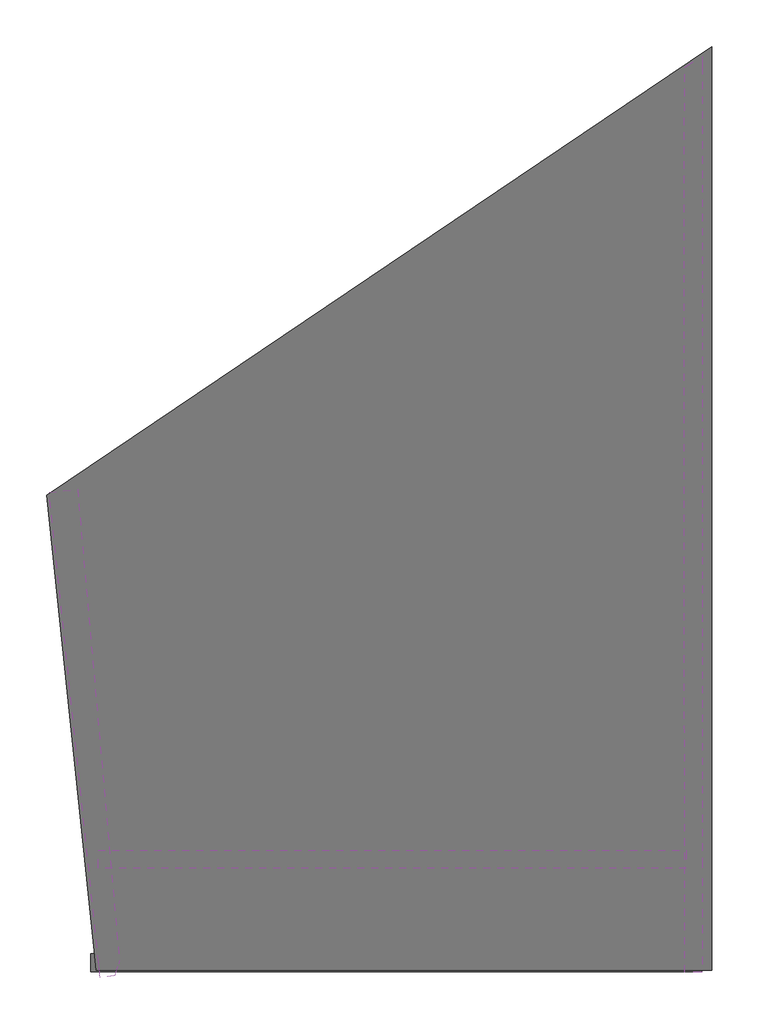
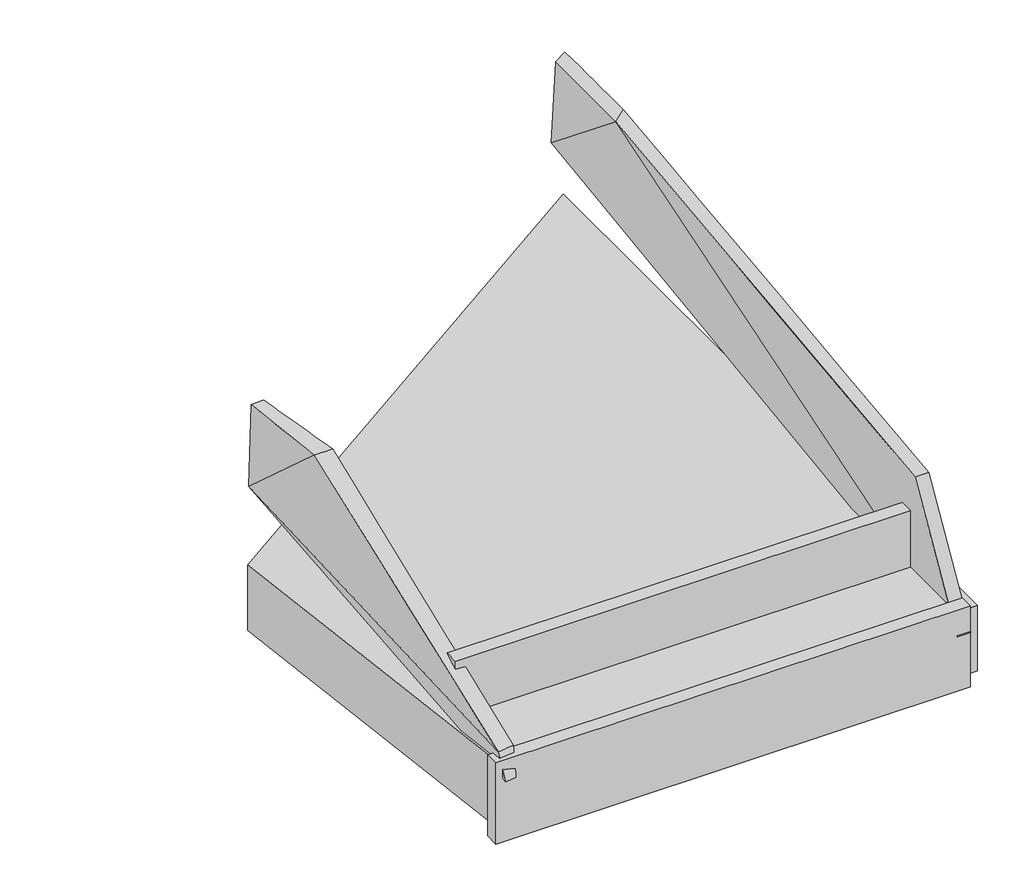
# One storey: 5 proxies.
"""IFC4 building model written with IfcOpenShell, lengths in millimetres."""

import ifcopenshell
import ifcopenshell.guid

model = None  # the IFC model being written
_history = None  # IfcOwnerHistory: only IFC2X3 demands one
_inside = {}  # id of a spatial element -> (the spatial element, [elements in it])
_under = {}  # id of a project, library or spatial element -> (it, [spatial elements below it])
_declared = {}  # id of a project -> (the project, [libraries it declares])
_typed = {}  # id of a type object -> (the type object, [elements of that type])
_made_of = {}  # id of a material, layer set ... -> (it, [elements and type objects made of it])


def new_model(schema):
    """Start an empty IFC model of exactly this schema.

    Asked for "IFC4X3", IfcOpenShell would pick the latest addendum, in which some entities
    have other attributes; the version numbers below select the first issue.
    IFC2X3 requires an IfcOwnerHistory on every rooted entity: one is made here for all.
    """
    global model, _history
    if schema == "IFC4X3":
        model = ifcopenshell.file(schema_version=(4, 3, 0, 0))
    else:
        model = ifcopenshell.file(schema=schema)
    _inside.clear()
    _under.clear()
    _declared.clear()
    _typed.clear()
    _made_of.clear()
    _history = None
    if model.schema == "IFC2X3":
        org = make("IfcOrganization", Name="unknown")
        user = make(
            "IfcPersonAndOrganization",
            ThePerson=make("IfcPerson", FamilyName="unknown"),
            TheOrganization=org,
        )
        app = make(
            "IfcApplication",
            ApplicationDeveloper=org,
            Version="unknown",
            ApplicationFullName="unknown",
            ApplicationIdentifier="unknown",
        )
        _history = make(
            "IfcOwnerHistory",
            OwningUser=user,
            OwningApplication=app,
            ChangeAction="ADDED",
            CreationDate=0,
        )
    return model


def make(cls, **values):
    """One entity of the class cls with the attributes given. An attribute that is None is left unset."""
    return model.create_entity(
        cls, **{name: value for name, value in values.items() if value is not None}
    )


def rooted(cls, **values):
    """An entity with a GlobalId (a new one), such as an element, a storey or a relation."""
    return make(cls, GlobalId=ifcopenshell.guid.new(), OwnerHistory=_history, **values)


def si_unit(unit_type, name, prefix=None):
    """IfcSIUnit, for example si_unit("LENGTHUNIT", "METRE", prefix="MILLI")."""
    return make("IfcSIUnit", UnitType=unit_type, Prefix=prefix, Name=name)


def assignment(units):
    """IfcUnitAssignment: the units of a project."""
    return None if units is None else make("IfcUnitAssignment", Units=units)


def point(xyz):
    """IfcCartesianPoint."""
    return None if xyz is None else make("IfcCartesianPoint", Coordinates=xyz)


def direction(xyz):
    """IfcDirection."""
    return None if xyz is None else make("IfcDirection", DirectionRatios=xyz)


def frame(location, z_axis=None, x_axis=None):
    """IfcAxis2Placement3D, a coordinate frame: its origin and axes. An axis left out is left unset."""
    return make(
        "IfcAxis2Placement3D",
        Location=point(location),
        Axis=direction(z_axis),
        RefDirection=direction(x_axis),
    )


def origin():
    """The frame at (0, 0, 0) with its axes left unset."""
    return frame((0.0, 0.0, 0.0))


def place(relative_to, where):
    """IfcLocalPlacement: puts the frame where relative to a parent placement (None: the world)."""
    return make(
        "IfcLocalPlacement", PlacementRelTo=relative_to, RelativePlacement=where
    )


def context(
    kind, dimensions, precision=None, world=None, true_north=None, identifier=None
):
    """IfcGeometricRepresentationContext, for example the 3D "Model" context."""
    return make(
        "IfcGeometricRepresentationContext",
        ContextIdentifier=identifier,
        ContextType=kind,
        CoordinateSpaceDimension=dimensions,
        Precision=precision,
        WorldCoordinateSystem=world,
        TrueNorth=true_north,
    )


def project(units=None, contexts=None):
    """IfcProject with its units and contexts."""
    return rooted(
        "IfcProject",
        Name="project",
        RepresentationContexts=contexts,
        UnitsInContext=assignment(units),
    )


def spatial(cls, under=None, at=None, **own):
    """A site, building, storey or space (cls), placed at a placement, below another one or the project."""
    s = rooted(cls, ObjectPlacement=at, **own)
    if under is not None:
        _under.setdefault(under.id(), (under, []))[1].append(s)
    return s


def polyline(points):
    """IfcPolyline through the points."""
    return make("IfcPolyline", Points=[point(p) for p in points])


def outline(outer, holes=None, kind="AREA"):
    """IfcArbitraryClosedProfileDef: a profile drawn as a closed curve; with holes, ...WithVoids."""
    if holes is None:
        return make("IfcArbitraryClosedProfileDef", ProfileType=kind, OuterCurve=outer)
    return make(
        "IfcArbitraryProfileDefWithVoids",
        ProfileType=kind,
        OuterCurve=outer,
        InnerCurves=holes,
    )


def extrude(swept, where, along, depth):
    """IfcExtrudedAreaSolid: the profile swept, set in the frame where, extruded along a direction by depth."""
    return make(
        "IfcExtrudedAreaSolid",
        SweptArea=swept,
        Position=where,
        ExtrudedDirection=direction(along),
        Depth=depth,
    )


def shape(context_of_items, identifier, shape_type, items):
    """IfcShapeRepresentation: the items that make up one representation, for example the "Body"."""
    return make(
        "IfcShapeRepresentation",
        ContextOfItems=context_of_items,
        RepresentationIdentifier=identifier,
        RepresentationType=shape_type,
        Items=items,
    )


def source(mapping_origin, context_of_items, identifier, shape_type, items):
    """IfcRepresentationMap: a shape defined once, which mapped items show again and again."""
    return make(
        "IfcRepresentationMap",
        MappingOrigin=mapping_origin,
        MappedRepresentation=shape(context_of_items, identifier, shape_type, items),
    )


def transform(
    local_origin,
    x_axis=None,
    y_axis=None,
    z_axis=None,
    scale=None,
    scale2=None,
    scale3=None,
    uniform=True,
):
    """IfcCartesianTransformationOperator3D, or its non-uniform kind. x_axis, y_axis, z_axis: its Axis1, 2, 3."""
    if uniform:
        return make(
            "IfcCartesianTransformationOperator3D",
            Axis1=direction(x_axis),
            Axis2=direction(y_axis),
            LocalOrigin=point(local_origin),
            Scale=scale,
            Axis3=direction(z_axis),
        )
    return make(
        "IfcCartesianTransformationOperator3DnonUniform",
        Axis1=direction(x_axis),
        Axis2=direction(y_axis),
        LocalOrigin=point(local_origin),
        Scale=scale,
        Axis3=direction(z_axis),
        Scale2=scale2,
        Scale3=scale3,
    )


def mapped(mapping_source, mapping_target):
    """IfcMappedItem: shows the shape of a source again, moved by a transform."""
    return make(
        "IfcMappedItem", MappingSource=mapping_source, MappingTarget=mapping_target
    )


def made_of(thing, what):
    """Note that an element or type object is made of a material, layer set ...; save() writes the relation."""
    if what is not None:
        _made_of.setdefault(what.id(), (what, []))[1].append(thing)
    return thing


def element(
    cls,
    number,
    at=None,
    inside=None,
    cuts=None,
    type_object=None,
    material=None,
    context=None,
    identifier="Body",
    shape_type=None,
    held_by="IfcProductDefinitionShape",
    body=None,
    shapes=None,
    **own,
):
    """One element of the class cls, such as IfcWall. Its Tag is "e" and its number.

    at: its placement. inside: the storey or other place that contains it. cuts: it is an
    opening in that element (IfcRelVoidsElement). A single representation is given by context,
    identifier, shape_type and body (its items); several are given by shapes. held_by: the class
    of the entity that holds the representations. save() writes the other relations.
    """
    e = rooted(cls, Tag="e%d" % number, ObjectPlacement=at, **own)
    if body is not None:
        shapes = [shape(context, identifier, shape_type, body)]
    if shapes is not None:
        e.Representation = make(held_by, Representations=shapes)
    if inside is not None:
        _inside.setdefault(inside.id(), (inside, []))[1].append(e)
    if cuts is not None:
        rooted(
            "IfcRelVoidsElement", RelatingBuildingElement=cuts, RelatedOpeningElement=e
        )
    if type_object is not None:
        _typed.setdefault(type_object.id(), (type_object, []))[1].append(e)
    return made_of(e, material)


def aggregate(whole, parts):
    """IfcRelAggregates: a whole, such as a stair, and the parts it consists of."""
    return rooted("IfcRelAggregates", RelatingObject=whole, RelatedObjects=parts)


def save(model, path):
    """Write the relations noted so far, then the file.

    IfcRelAggregates (storeys below a building ...), IfcRelContainedInSpatialStructure (elements
    in a storey), IfcRelDefinesByType, IfcRelAssociatesMaterial and IfcRelDeclares: one each for
    every whole, place, type object, material and project.
    """
    for whole, parts in _under.values():
        aggregate(whole, parts)
    for where, things in _inside.values():
        rooted(
            "IfcRelContainedInSpatialStructure",
            RelatedElements=things,
            RelatingStructure=where,
        )
    for kind, things in _typed.values():
        rooted("IfcRelDefinesByType", RelatedObjects=things, RelatingType=kind)
    for what, things in _made_of.values():
        rooted("IfcRelAssociatesMaterial", RelatedObjects=things, RelatingMaterial=what)
    for by, libraries in _declared.values():
        rooted("IfcRelDeclares", RelatingContext=by, RelatedDefinitions=libraries)
    model.write(path)


def plane_surface(at):
    """IfcPlane: the flat surface through the origin of the frame at, square to its z axis."""
    return make("IfcPlane", Position=at)


def spline_surface(u_degree, v_degree, points, u_multiplicities, v_multiplicities, u_knots, v_knots, weights=None):
    """IfcBSplineSurfaceWithKnots; with weights, IfcRationalBSplineSurfaceWithKnots. points: one row for each step in u."""
    own = dict(
        UDegree=u_degree,
        VDegree=v_degree,
        ControlPointsList=[[point(p) for p in row] for row in points],
        SurfaceForm="UNSPECIFIED",
        UClosed=False,
        VClosed=False,
        SelfIntersect=False,
        UMultiplicities=u_multiplicities,
        VMultiplicities=v_multiplicities,
        UKnots=u_knots,
        VKnots=v_knots,
        KnotSpec="UNSPECIFIED",
    )
    if weights is None:
        return make("IfcBSplineSurfaceWithKnots", **own)
    return make("IfcRationalBSplineSurfaceWithKnots", WeightsData=weights, **own)


def advanced_brep(points, edges, surfaces, faces):
    """IfcAdvancedBrep: a solid bounded by faces that lie on surfaces and meet in shared edges.

    An edge is (start, end): straight between two places in points (the first is 0);
    or (start, end, curve); or (start, end, curve, False) where it runs against its curve.
    A face is (place in surfaces, loops), or (place, loops, False) where it looks against
    its surface's normal. A loop lists edges by number (the first is 1), with a minus sign
    where the edge is run from its end to its start. The first loop is the outer one.
    """
    corners = [point(p) for p in points]
    vertices = [make("IfcVertexPoint", VertexGeometry=c) for c in corners]
    made = []
    for start, end, *more in edges:
        made.append(
            make(
                "IfcEdgeCurve",
                EdgeStart=vertices[start],
                EdgeEnd=vertices[end],
                EdgeGeometry=more[0] if more else make("IfcPolyline", Points=[corners[start], corners[end]]),
                SameSense=more[1] if len(more) > 1 else True,
            )
        )
    hull = []
    for where, loops, *sense in faces:
        bounds = []
        for j, loop in enumerate(loops):
            ring = [make("IfcOrientedEdge", EdgeElement=made[abs(k) - 1], Orientation=k > 0) for k in loop]
            bounds.append(
                make(
                    "IfcFaceOuterBound" if j == 0 else "IfcFaceBound",
                    Bound=make("IfcEdgeLoop", EdgeList=ring),
                    Orientation=True,
                )
            )
        hull.append(make("IfcAdvancedFace", Bounds=bounds, FaceSurface=surfaces[where], SameSense=sense[0] if sense else True))
    return make("IfcAdvancedBrep", Outer=make("IfcClosedShell", CfsFaces=hull))


def topography_6_topography_1_ed09c014(model_context):
    return source(origin(), model_context, "Body", "SweptSolid", [
        extrude(outline(polyline([(136325.9552311, 39054.0681482), (134220.0017656, 59090.8769425), (162308.6227529, 78036.8910248), (162308.6227529, 39054.0681482), (136325.9552311, 39054.0681482)])), frame((0.0, 0.0, -10500.0), z_axis=(0.0, 0.0, 1.0), x_axis=(1.0, 0.0, 0.0)), (0.0, 0.0, 1.0), 3770.0),
    ])


model = new_model("IFC4")

# Units and contexts
model_context = context("Model", 3, world=origin())
ifc_project = project(units=[si_unit("LENGTHUNIT", "METRE", prefix="MILLI")], contexts=[model_context])

# Site, building, storey
site = spatial("IfcSite", under=ifc_project)
building = spatial("IfcBuilding", under=site)
storey = spatial("IfcBuildingStorey", under=building, Name="ALT KOT", Elevation=-10500.0)

# Proxies
placement = place(None, origin())
element("IfcBuildingElementProxy", 1, Name="Mass 1 : Mass 1", ObjectType="Mass 1 : Mass 1", at=placement, inside=storey, context=model_context, shape_type="AdvancedBrep", body=[
    advanced_brep(
    [(161372.4922022, 42934.3784589, -1314.7586173), (161372.4922022, 38961.5454586, -8080.0303991), (162116.7322799, 38961.5454586, -8080.0303991), (162116.7322799, 42934.3784589, -1314.7586173), (161372.4922022, 77166.0470906, -2849.8677352), (162116.7322799, 77615.0485221, -2810.4563106), (161372.4922022, 76734.4523501, 2067.1495608), (162116.7322799, 77183.5173991, 2100.2004181), (161354.0623385, 71052.3578898, 2069.0620598), (162098.3024161, 71637.2194872, 2155.5942168)],
    [
        (0, 1),
        (1, 2),
        (2, 3),
        (3, 0),
        (1, 4),
        (4, 5),
        (5, 2),
        (4, 6),
        (6, 7),
        (7, 5),
        (8, 0),
        (3, 9),
        (9, 8),
        (6, 8),
        (9, 7),
        (5, 9),
        (9, 2),
        (8, 1),
        (4, 8),
    ],
    [
        plane_surface(frame((161372.4922022, 40947.9619588, -4697.3945082), z_axis=(0.0, -0.8623093399622475, 0.5063818738994055), x_axis=(0.0, -0.5063818738994055, -0.8623093399622475))),
        spline_surface(1, 1, [[(161372.4922022, 38961.5454586, -8080.0303991), (162116.7322799, 38961.5454586, -8080.0303991)], [(161372.4922022, 77166.0470906, -2849.8677352), (162116.7322799, 77615.0485221, -2810.4563106)]], [2, 2], [2, 2], [0.0, 1.0], [0.0, 1.0]),
        spline_surface(1, 1, [[(161372.4922022, 77166.0470906, -2849.8677352), (162116.7322799, 77615.0485221, -2810.4563106)], [(161372.4922022, 76734.4523501, 2067.1495608), (162116.7322799, 77183.5173991, 2100.2004181)]], [2, 2], [2, 2], [0.0, 1.0], [0.0, 1.0]),
        spline_surface(1, 1, [[(161354.0623385, 71052.3578898, 2069.0620598), (162098.3024161, 71637.2194872, 2155.5942168)], [(161372.4922022, 42934.3784589, -1314.7586173), (162116.7322799, 42934.3784589, -1314.7586173)]], [2, 2], [2, 2], [0.0, 1.0], [0.0, 1.0]),
        spline_surface(1, 1, [[(161372.4922022, 76734.4523501, 2067.1495608), (162116.7322799, 77183.5173991, 2100.2004181)], [(161354.0623385, 71052.3578898, 2069.0620598), (162098.3024161, 71637.2194872, 2155.5942168)]], [2, 2], [2, 2], [0.0, 1.0], [0.0, 1.0]),
        plane_surface(frame((162110.588992, 62737.9378226, -2911.630831), z_axis=(0.9999948239010785, -0.00043461392743272516, 0.003187990242341914), x_axis=(-0.00237146360557062, -0.769197437953617, 0.6390067899529387))),
        plane_surface(frame((162110.588992, 51177.7144682, -2413.0649332), z_axis=(0.9999996787763593, 0.0006911651041640725, -0.00040587926444148287), x_axis=(0.0, -0.5063818738994055, -0.8623093399622475))),
        plane_surface(frame((162110.588992, 75478.5951361, 481.7794414), z_axis=(0.9999944267597863, -0.003325813142761698, -0.00029226068114899156), x_axis=(0.0, -0.08753910828298744, 0.9961610836210274))),
        plane_surface(frame((161366.3489143, 50982.7606024, -2441.9089855), z_axis=(-0.9999996655122543, -0.000705290700216393, 0.00041417436860819237), x_axis=(0.0005475714268804593, -0.9534531653964613, -0.3015406466150139))),
        plane_surface(frame((161366.3489143, 74984.2857768, 428.7812951), z_axis=(-0.999994699061132, 0.0032435769431798825, 0.0002847073062190215), x_axis=(0.0032434810641479525, 0.9999946832575457, -0.00033658168034393757))),
        plane_surface(frame((161366.3489143, 62393.316813, -2953.6120248), z_axis=(-0.9999947778414309, 0.0004383370135836915, -0.0032018979574588782), x_axis=(0.0023486891283887473, 0.7791243351897017, -0.6268650205383799))),
    ],
    [
        (0, [[1, 2, 3, 4]]),
        (1, [[5, 6, 7, -2]]),
        (2, [[8, 9, 10, -6]]),
        (3, [[11, -4, 12, 13]]),
        (4, [[14, -13, 15, -9]]),
        (5, [[16, 17, -7]]),
        (6, [[-3, -17, -12]]),
        (7, [[-10, -15, -16]]),
        (8, [[18, -1, -11]]),
        (9, [[-14, -8, 19]]),
        (10, [[-19, -5, -18]]),
    ],
),
])
element("IfcBuildingElementProxy", 2, Name="Mass 2 : Mass 2", ObjectType="Mass 2 : Mass 2", at=placement, inside=storey, context=model_context, shape_type="AdvancedBrep", body=[
    advanced_brep(
    [(135744.5091033, 59344.8309753, -2330.8855734), (137300.9488587, 38804.2814499, -7636.4184524), (136701.0552394, 38741.2300898, -7636.4184524), (134548.8239959, 59218.3425303, -2321.0250212), (137511.2980734, 39436.4761601, -6265.0150057), (136637.7167334, 39343.8557195, -6260.9626553), (136174.3983016, 54114.4522532, 2341.4885295), (135171.9120251, 54093.7487133, 2378.6225099), (135362.7132451, 59203.5859013, 2357.4684572), (134642.9020412, 59126.9425001, 2390.5500872)],
    [
        (0, 1),
        (1, 2),
        (2, 3),
        (3, 0),
        (1, 4),
        (4, 5),
        (5, 2),
        (4, 6),
        (6, 7),
        (7, 5),
        (8, 0),
        (3, 9),
        (9, 8),
        (7, 3),
        (3, 5),
        (7, 9),
        (6, 8),
        (4, 0),
        (0, 6),
    ],
    [
        spline_surface(1, 1, [[(135744.5091033, 59344.8309753, -2330.8855734), (134548.8239959, 59218.3425303, -2321.0250212)], [(137300.9488587, 38804.2814499, -7636.4184524), (136701.0552394, 38741.2300898, -7636.4184524)]], [2, 2], [2, 2], [0.0, 1.0], [0.0, 1.0]),
        spline_surface(1, 1, [[(137300.9488587, 38804.2814499, -7636.4184524), (136701.0552394, 38741.2300898, -7636.4184524)], [(137511.2980734, 39436.4761601, -6265.0150057), (136637.7167334, 39343.8557195, -6260.9626553)]], [2, 2], [2, 2], [0.0, 1.0], [0.0, 1.0]),
        spline_surface(1, 1, [[(137511.2980734, 39436.4761601, -6265.0150057), (136637.7167334, 39343.8557195, -6260.9626553)], [(136174.3983016, 54114.4522532, 2341.4885295), (135171.9120251, 54093.7487133, 2378.6225099)]], [2, 2], [2, 2], [0.0, 1.0], [0.0, 1.0]),
        spline_surface(1, 1, [[(135362.7132451, 59203.5859013, 2357.4684572), (134642.9020412, 59126.9425001, 2390.5500872)], [(135744.5091033, 59344.8309753, -2330.8855734), (134548.8239959, 59218.3425303, -2321.0250212)]], [2, 2], [2, 2], [0.0, 1.0], [0.0, 1.0]),
        plane_surface(frame((135452.8175848, 50885.3156544, -2067.7883889), z_axis=(-0.9941075979509935, -0.10739750594369274, 0.014692154817472214), x_axis=(-0.08543657456791878, 0.8597191191091914, 0.5035708768030739))),
        plane_surface(frame((134787.879354, 57479.6779146, 816.049192), z_axis=(-0.9943594675733274, -0.10455363650483235, 0.017826562789962475), x_axis=(0.08925298316439714, -0.734062065434937, 0.67319149510793))),
        spline_surface(1, 1, [[(136174.3983016, 54114.4522532, 2341.4885295), (135171.9120251, 54093.7487133, 2378.6225099)], [(135362.7132451, 59203.5859013, 2357.4684572), (134642.9020412, 59126.9425001, 2390.5500872)]], [2, 2], [2, 2], [0.0, 1.0], [0.0, 1.0]),
        plane_surface(frame((136476.7351594, 50965.2531295, -2084.8040165), z_axis=(0.9961707928177188, 0.08722339500488269, 0.005985891808217368), x_axis=(0.07832979268791743, -0.859991787456988, -0.5042604179231231))),
        plane_surface(frame((135760.5402167, 57554.2897099, 789.3571378), z_axis=(0.9839984898125396, 0.1566751821340282, 0.08485198494973899), x_axis=(0.1575022810417032, -0.9875137550892158, -0.003100802518184594))),
        plane_surface(frame((135962.5319895, 45767.8094465, -5406.1353763), z_axis=(-0.9945218953682737, -0.1045284632676509, 0.0), x_axis=(-0.1025543164477561, 0.9757391430376474, 0.19343147862251162))),
        plane_surface(frame((136852.2520118, 45861.8628618, -5410.7730105), z_axis=(0.9699808967252863, 0.127056697108277, -0.20734911552245647), x_axis=(-0.13796240818906627, -0.4146395544410477, -0.8994667385843698))),
    ],
    [
        (0, [[1, 2, 3, 4]]),
        (1, [[5, 6, 7, -2]]),
        (2, [[8, 9, 10, -6]]),
        (3, [[11, -4, 12, 13]]),
        (4, [[-10, 14, 15]]),
        (5, [[-14, 16, -12]]),
        (6, [[17, -13, -16, -9]]),
        (7, [[-8, 18, 19]]),
        (8, [[-17, -19, -11]]),
        (9, [[-15, -3, -7]]),
        (10, [[-5, -1, -18]]),
    ],
),
])
element("IfcBuildingElementProxy", 3, Name="Mass 3 : Mass 3", ObjectType="Mass 3 : Mass 3", at=placement, inside=storey, context=model_context, shape_type="SweptSolid", body=[
    extrude(outline(polyline([(136306.1772957, 39752.4836972), (162093.5425765, 39752.4836972), (162093.5425765, 38982.5949075), (136306.1772957, 38982.5949075), (136306.1772957, 39752.4836972)])), frame((0.0, 0.0, -11238.6614816), z_axis=(0.0, 0.0, 1.0), x_axis=(1.0, 0.0, 0.0)), (0.0, 0.0, 1.0), 4671.5466692),
])
element("IfcBuildingElementProxy", 4, Name="Mass 5 : Mass 3", ObjectType="Mass 5 : Mass 3", at=placement, inside=storey, context=model_context, shape_type="SweptSolid", body=[
    extrude(outline(polyline([(136620.3193722, 44112.437321), (161444.6398615, 44112.437321), (161444.6398615, 43342.5485313), (136620.3193722, 43342.5485313), (136620.3193722, 44112.437321)])), frame((0.0, 0.0, -8213.1140936), z_axis=(0.0, 0.0, 1.0), x_axis=(1.0, 0.0, 0.0)), (0.0, 0.0, 1.0), 4737.9354369),
])
topography_6_topography_1_shape = topography_6_topography_1_ed09c014(model_context)
element("IfcBuildingElementProxy", 5, Name="Topography 6 : Topography 1", ObjectType="Topography 6 : Topography 1", at=placement, inside=storey, context=model_context, shape_type="MappedRepresentation", body=[
    mapped(topography_6_topography_1_shape, transform((217.3446501, 0.0, 0.0), x_axis=(1.0, 0.0, 0.0), y_axis=(0.0, 1.0, 0.0), z_axis=(0.0, 0.0, 1.0))),
])

save(model, "model.ifc")

# Revit data of these elements
# Project information
#   Organization Name = "Organization Name"
#   Organization Description = "Organization Description"
#   Building Name = "Building Name"
#   Project Issue Date = "Issue Date"
#   Project Status = "Project Status"
#   Client Name = "Client Name"
#   Project Address = "Enter address here\nAddress Line 2"
#   Project Name = "Project Name"
#   Project Number = "Project Number"
# Grids (mm)
#   "3": line (130114.425, 63456.848) -> (166514.796, 63456.848)
#   "1": line (130114.425, 73456.848) -> (166514.796, 73456.848)
#   "2": line (130114.425, 68456.848) -> (166514.796, 68456.848)
#   "A": line (133450.757, 36925.861) -> (133450.757, 77450.132)
#   "8": line (130114.425, 38456.848) -> (166514.796, 38456.848)
#   "7": line (130114.425, 43456.848) -> (166514.796, 43456.848)
#   "6": line (130114.425, 48456.848) -> (166514.796, 48456.848)
#   "5": line (130114.425, 53456.848) -> (166514.796, 53456.848)
#   "4": line (130114.425, 58456.848) -> (166514.796, 58456.848)
#   "B": line (138450.757, 36925.861) -> (138450.757, 77450.132)
#   "C": line (143450.757, 36925.861) -> (143450.757, 77450.132)
#   "D": line (148450.757, 36925.861) -> (148450.757, 77450.132)
#   "E": line (153450.757, 36925.861) -> (153450.757, 77450.132)
#   "F": line (158450.757, 36925.861) -> (158450.757, 77450.132)
#   "G": line (163450.757, 36925.861) -> (163450.757, 77450.132)
# Element 1 (IfcBuildingElementProxy, "Mass 1 : Mass 1")
#   Phase Created = istinat
#   Materials on its faces: "Gravel"
# Element 2 (IfcBuildingElementProxy, "Mass 2 : Mass 2")
#   Phase Created = istinat
#   Materials on its faces: "Gravel"
# Element 3 (IfcBuildingElementProxy, "Mass 3 : Mass 3")
#   Phase Created = istinat
#   Materials on its faces: "Gravel"
# Element 4 (IfcBuildingElementProxy, "Mass 5 : Mass 3")
#   Phase Created = istinat
#   Materials on its faces: "Gravel"
# Element 5 (IfcBuildingElementProxy, "Topography 6 : Topography 1")
#   Phase Created = Çekmeler
#   Materials on its faces: "Grass"
# Materials
#   "Gravel": class "Generic", colour RGB 183 182 178, transparency 0, Description = "Crushed stone or gravel", Cost = 0
#   "Grass": class "Generic", colour RGB 0 185 92, transparency 0, Description = "Physical material.", Cost = 0
